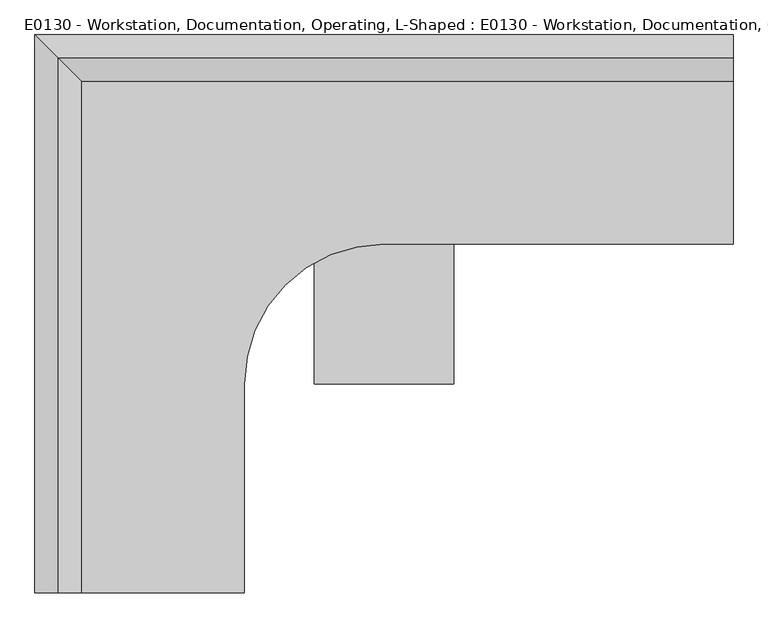
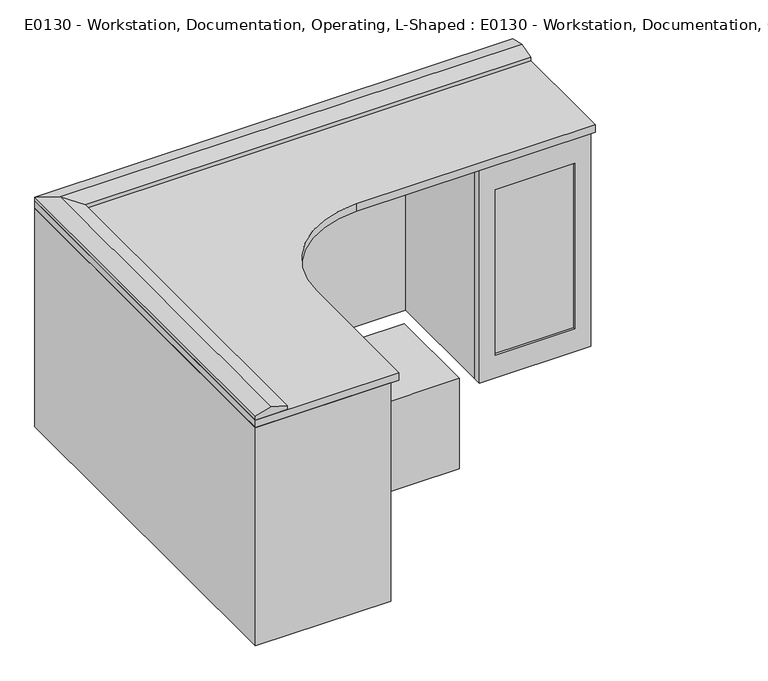
"""IFC4 building model written with IfcOpenShell, lengths in millimetres: proxy geometry, E0130 - Workstation, Documentation, Operating, L-Shaped : E0130 - Workstation, Documentation, Operating, L-Shaped."""

import ifcopenshell
import ifcopenshell.guid

model = None  # the IFC model being written
_history = None  # IfcOwnerHistory: only IFC2X3 demands one
_inside = {}  # id of a spatial element -> (the spatial element, [elements in it])
_under = {}  # id of a project, library or spatial element -> (it, [spatial elements below it])
_declared = {}  # id of a project -> (the project, [libraries it declares])
_typed = {}  # id of a type object -> (the type object, [elements of that type])
_made_of = {}  # id of a material, layer set ... -> (it, [elements and type objects made of it])


def new_model(schema):
    """Start an empty IFC model of exactly this schema.

    Asked for "IFC4X3", IfcOpenShell would pick the latest addendum, in which some entities
    have other attributes; the version numbers below select the first issue.
    IFC2X3 requires an IfcOwnerHistory on every rooted entity: one is made here for all.
    """
    global model, _history
    if schema == "IFC4X3":
        model = ifcopenshell.file(schema_version=(4, 3, 0, 0))
    else:
        model = ifcopenshell.file(schema=schema)
    _inside.clear()
    _under.clear()
    _declared.clear()
    _typed.clear()
    _made_of.clear()
    _history = None
    if model.schema == "IFC2X3":
        org = make("IfcOrganization", Name="unknown")
        user = make(
            "IfcPersonAndOrganization",
            ThePerson=make("IfcPerson", FamilyName="unknown"),
            TheOrganization=org,
        )
        app = make(
            "IfcApplication",
            ApplicationDeveloper=org,
            Version="unknown",
            ApplicationFullName="unknown",
            ApplicationIdentifier="unknown",
        )
        _history = make(
            "IfcOwnerHistory",
            OwningUser=user,
            OwningApplication=app,
            ChangeAction="ADDED",
            CreationDate=0,
        )
    return model


def make(cls, **values):
    """One entity of the class cls with the attributes given. An attribute that is None is left unset."""
    return model.create_entity(
        cls, **{name: value for name, value in values.items() if value is not None}
    )


def rooted(cls, **values):
    """An entity with a GlobalId (a new one), such as an element, a storey or a relation."""
    return make(cls, GlobalId=ifcopenshell.guid.new(), OwnerHistory=_history, **values)


def si_unit(unit_type, name, prefix=None):
    """IfcSIUnit, for example si_unit("LENGTHUNIT", "METRE", prefix="MILLI")."""
    return make("IfcSIUnit", UnitType=unit_type, Prefix=prefix, Name=name)


def assignment(units):
    """IfcUnitAssignment: the units of a project."""
    return None if units is None else make("IfcUnitAssignment", Units=units)


def point(xyz):
    """IfcCartesianPoint."""
    return None if xyz is None else make("IfcCartesianPoint", Coordinates=xyz)


def direction(xyz):
    """IfcDirection."""
    return None if xyz is None else make("IfcDirection", DirectionRatios=xyz)


def frame(location, z_axis=None, x_axis=None):
    """IfcAxis2Placement3D, a coordinate frame: its origin and axes. An axis left out is left unset."""
    return make(
        "IfcAxis2Placement3D",
        Location=point(location),
        Axis=direction(z_axis),
        RefDirection=direction(x_axis),
    )


def frame_2d(location, x_axis=None):
    """IfcAxis2Placement2D, a coordinate frame in the plane: its origin and x axis."""
    return make(
        "IfcAxis2Placement2D", Location=point(location), RefDirection=direction(x_axis)
    )


def origin():
    """The frame at (0, 0, 0) with its axes left unset."""
    return frame((0.0, 0.0, 0.0))


def origin_with_axes():
    """The frame at (0, 0, 0) with the z axis (0, 0, 1) and the x axis (1, 0, 0) written out."""
    return frame((0.0, 0.0, 0.0), z_axis=(0.0, 0.0, 1.0), x_axis=(1.0, 0.0, 0.0))


def place(relative_to, where):
    """IfcLocalPlacement: puts the frame where relative to a parent placement (None: the world)."""
    return make(
        "IfcLocalPlacement", PlacementRelTo=relative_to, RelativePlacement=where
    )


def context(
    kind, dimensions, precision=None, world=None, true_north=None, identifier=None
):
    """IfcGeometricRepresentationContext, for example the 3D "Model" context."""
    return make(
        "IfcGeometricRepresentationContext",
        ContextIdentifier=identifier,
        ContextType=kind,
        CoordinateSpaceDimension=dimensions,
        Precision=precision,
        WorldCoordinateSystem=world,
        TrueNorth=true_north,
    )


def project(units=None, contexts=None):
    """IfcProject with its units and contexts."""
    return rooted(
        "IfcProject",
        Name="project",
        RepresentationContexts=contexts,
        UnitsInContext=assignment(units),
    )


def spatial(cls, under=None, at=None, **own):
    """A site, building, storey or space (cls), placed at a placement, below another one or the project."""
    s = rooted(cls, ObjectPlacement=at, **own)
    if under is not None:
        _under.setdefault(under.id(), (under, []))[1].append(s)
    return s


def polyline(points):
    """IfcPolyline through the points."""
    return make("IfcPolyline", Points=[point(p) for p in points])


def circle_curve(where, radius):
    """IfcCircle in the frame where."""
    return make("IfcCircle", Position=where, Radius=radius)


def trimmed(basis, trim1, trim2, sense, master):
    """IfcTrimmedCurve: the piece of a basis curve between two trims."""
    return make(
        "IfcTrimmedCurve",
        BasisCurve=basis,
        Trim1=trim1,
        Trim2=trim2,
        SenseAgreement=sense,
        MasterRepresentation=master,
    )


def segment(curve, same_sense, transition):
    """IfcCompositeCurveSegment."""
    return make(
        "IfcCompositeCurveSegment",
        Transition=transition,
        SameSense=same_sense,
        ParentCurve=curve,
    )


def composite_curve(segments, self_intersect=None):
    """IfcCompositeCurve: segments joined end to end."""
    return make("IfcCompositeCurve", Segments=segments, SelfIntersect=self_intersect)


def outline(outer, holes=None, kind="AREA"):
    """IfcArbitraryClosedProfileDef: a profile drawn as a closed curve; with holes, ...WithVoids."""
    if holes is None:
        return make("IfcArbitraryClosedProfileDef", ProfileType=kind, OuterCurve=outer)
    return make(
        "IfcArbitraryProfileDefWithVoids",
        ProfileType=kind,
        OuterCurve=outer,
        InnerCurves=holes,
    )


def extrude(swept, where, along, depth):
    """IfcExtrudedAreaSolid: the profile swept, set in the frame where, extruded along a direction by depth."""
    return make(
        "IfcExtrudedAreaSolid",
        SweptArea=swept,
        Position=where,
        ExtrudedDirection=direction(along),
        Depth=depth,
    )


def faces_of(points, faces, orient=None, outer=None):
    """IfcFace entities. A face is a list of loops; a loop is a list of indices into points, from 0.

    orient and outer hold one flag for each loop. By default every Orientation is true, the
    first loop of a face is its IfcFaceOuterBound and the others are IfcFaceBound.
    """
    made = []
    for i, loops in enumerate(faces):
        bounds = []
        for j, loop in enumerate(loops):
            is_outer = j == 0 if outer is None else outer[i][j]
            bounds.append(
                make(
                    "IfcFaceOuterBound" if is_outer else "IfcFaceBound",
                    Bound=make("IfcPolyLoop", Polygon=[points[k] for k in loop]),
                    Orientation=True if orient is None else orient[i][j],
                )
            )
        made.append(make("IfcFace", Bounds=bounds))
    return made


def faceted_brep(points, faces, orient=None, outer=None, voids=None):
    """IfcFacetedBrep: a solid bounded by flat faces; with voids (closed shells), ...WithVoids."""
    shared = [point(p) for p in points]
    hull = make("IfcClosedShell", CfsFaces=faces_of(shared, faces, orient, outer))
    if voids is None:
        return make("IfcFacetedBrep", Outer=hull)
    return make(
        "IfcFacetedBrepWithVoids",
        Outer=hull,
        Voids=[
            make(cls, CfsFaces=faces_of(shared, fs, o, b)) for cls, fs, o, b in voids
        ],
    )


def shape(context_of_items, identifier, shape_type, items):
    """IfcShapeRepresentation: the items that make up one representation, for example the "Body"."""
    return make(
        "IfcShapeRepresentation",
        ContextOfItems=context_of_items,
        RepresentationIdentifier=identifier,
        RepresentationType=shape_type,
        Items=items,
    )


def source(mapping_origin, context_of_items, identifier, shape_type, items):
    """IfcRepresentationMap: a shape defined once, which mapped items show again and again."""
    return make(
        "IfcRepresentationMap",
        MappingOrigin=mapping_origin,
        MappedRepresentation=shape(context_of_items, identifier, shape_type, items),
    )


def transform(
    local_origin,
    x_axis=None,
    y_axis=None,
    z_axis=None,
    scale=None,
    scale2=None,
    scale3=None,
    uniform=True,
):
    """IfcCartesianTransformationOperator3D, or its non-uniform kind. x_axis, y_axis, z_axis: its Axis1, 2, 3."""
    if uniform:
        return make(
            "IfcCartesianTransformationOperator3D",
            Axis1=direction(x_axis),
            Axis2=direction(y_axis),
            LocalOrigin=point(local_origin),
            Scale=scale,
            Axis3=direction(z_axis),
        )
    return make(
        "IfcCartesianTransformationOperator3DnonUniform",
        Axis1=direction(x_axis),
        Axis2=direction(y_axis),
        LocalOrigin=point(local_origin),
        Scale=scale,
        Axis3=direction(z_axis),
        Scale2=scale2,
        Scale3=scale3,
    )


def mapped(mapping_source, mapping_target):
    """IfcMappedItem: shows the shape of a source again, moved by a transform."""
    return make(
        "IfcMappedItem", MappingSource=mapping_source, MappingTarget=mapping_target
    )


def made_of(thing, what):
    """Note that an element or type object is made of a material, layer set ...; save() writes the relation."""
    if what is not None:
        _made_of.setdefault(what.id(), (what, []))[1].append(thing)
    return thing


def element(
    cls,
    number,
    at=None,
    inside=None,
    cuts=None,
    type_object=None,
    material=None,
    context=None,
    identifier="Body",
    shape_type=None,
    held_by="IfcProductDefinitionShape",
    body=None,
    shapes=None,
    **own,
):
    """One element of the class cls, such as IfcWall. Its Tag is "e" and its number.

    at: its placement. inside: the storey or other place that contains it. cuts: it is an
    opening in that element (IfcRelVoidsElement). A single representation is given by context,
    identifier, shape_type and body (its items); several are given by shapes. held_by: the class
    of the entity that holds the representations. save() writes the other relations.
    """
    e = rooted(cls, Tag="e%d" % number, ObjectPlacement=at, **own)
    if body is not None:
        shapes = [shape(context, identifier, shape_type, body)]
    if shapes is not None:
        e.Representation = make(held_by, Representations=shapes)
    if inside is not None:
        _inside.setdefault(inside.id(), (inside, []))[1].append(e)
    if cuts is not None:
        rooted(
            "IfcRelVoidsElement", RelatingBuildingElement=cuts, RelatedOpeningElement=e
        )
    if type_object is not None:
        _typed.setdefault(type_object.id(), (type_object, []))[1].append(e)
    return made_of(e, material)


def aggregate(whole, parts):
    """IfcRelAggregates: a whole, such as a stair, and the parts it consists of."""
    return rooted("IfcRelAggregates", RelatingObject=whole, RelatedObjects=parts)


def save(model, path):
    """Write the relations noted so far, then the file.

    IfcRelAggregates (storeys below a building ...), IfcRelContainedInSpatialStructure (elements
    in a storey), IfcRelDefinesByType, IfcRelAssociatesMaterial and IfcRelDeclares: one each for
    every whole, place, type object, material and project.
    """
    for whole, parts in _under.values():
        aggregate(whole, parts)
    for where, things in _inside.values():
        rooted(
            "IfcRelContainedInSpatialStructure",
            RelatedElements=things,
            RelatingStructure=where,
        )
    for kind, things in _typed.values():
        rooted("IfcRelDefinesByType", RelatedObjects=things, RelatingType=kind)
    for what, things in _made_of.values():
        rooted("IfcRelAssociatesMaterial", RelatedObjects=things, RelatingMaterial=what)
    for by, libraries in _declared.values():
        rooted("IfcRelDeclares", RelatingContext=by, RelatedDefinitions=libraries)
    model.write(path)


def e0130_workstation_documentation_operating_l_shaped_e0130_dad7d897(model_context):
    return source(origin(), model_context, "Body", "SolidModel", [
        extrude(outline(polyline([(711.2, 184.9965826), (457.2, 184.9965826), (457.2, 193.8982967), (711.2, 193.8982967), (711.2, 184.9965826)])), frame((0.0, 0.0, 76.2), z_axis=(0.0, 0.0, 1.0), x_axis=(1.0, 0.0, 0.0)), (0.0, 0.0, 1.0), 558.8),
        extrude(outline(polyline([(736.6, 762.0), (736.6, 406.4), (0.0, 406.4), (0.0, 762.0), (736.6, 762.0)]), holes=[polyline([(635.0, 711.2), (76.2, 711.2), (76.2, 457.2), (635.0, 457.2), (635.0, 711.2)])]), frame((0.0, 177.8, 0.0), z_axis=(0.0, 1.0, 0.0), x_axis=(0.0, 0.0, 1.0)), (0.0, 0.0, 1.0), 25.4),
        faceted_brep([(-660.4, -609.6, 762.0), (-660.4, -609.6, 774.7), (-711.2, -609.6, 788.311819), (-762.0, -609.6, 774.7), (-762.0, -609.6, 762.0), (-762.0, 609.6, 762.0), (762.0, 609.6, 762.0), (762.0, 508.0, 762.0), (-660.4, 508.0, 762.0), (762.0, 609.6, 774.7), (762.0, 558.8, 788.311819), (762.0, 508.0, 774.7), (-660.4, 508.0, 774.7), (-711.2, 558.8, 788.311819), (-762.0, 609.6, 774.7)], [[[0, 1, 2, 3, 4]], [[0, 4, 5, 6, 7, 8]], [[7, 6, 9, 10, 11]], [[1, 0, 8, 12]], [[2, 1, 12, 13]], [[3, 2, 13, 14]], [[4, 3, 14, 5]], [[12, 8, 7, 11]], [[13, 12, 11, 10]], [[14, 13, 10, 9]], [[5, 14, 9, 6]]]),
        extrude(outline(polyline([(431.8, 558.8), (431.8, 203.2), (406.4, 203.2), (406.4, 584.2), (736.6, 584.2), (736.6, 558.8), (431.8, 558.8)])), origin_with_axes(), (0.0, 0.0, 1.0), 736.6),
        extrude(outline(polyline([(-762.0, 609.6), (762.0, 609.6), (762.0, 203.2), (736.6, 203.2), (736.6, 584.2), (-736.6, 584.2), (-736.6, -584.2), (-330.2, -584.2), (-330.2, -609.6), (-762.0, -609.6), (-762.0, 609.6)])), origin_with_axes(), (0.0, 0.0, 1.0), 736.6),
        extrude(outline(composite_curve([segment(polyline([(762.0, 609.6), (762.0, 152.4), (0.0, 152.4)]), True, "CONTINUOUS"), segment(trimmed(circle_curve(frame_2d((0.0, -152.4)), 304.8), [point((0.0, 152.4))], [point((-304.8, -152.4))], True, "CARTESIAN"), True, "CONTINUOUS"), segment(polyline([(-304.8, -152.4), (-304.8, -609.6), (-762.0, -609.6), (-762.0, 609.6), (762.0, 609.6)]), True, "CONTINUOUS")], self_intersect=False)), frame((0.0, 0.0, 736.6), z_axis=(0.0, 0.0, 1.0), x_axis=(1.0, 0.0, 0.0)), (0.0, 0.0, 1.0), 25.4),
        extrude(outline(polyline([(-152.4, 152.4), (152.4, 152.4), (152.4, -152.4), (-152.4, -152.4), (-152.4, 0.0), (-152.4, 152.4)])), origin_with_axes(), (0.0, 0.0, 1.0), 304.8),
    ])


if __name__ == "__main__":
    model = new_model("IFC4")
    model_context = context("Model", 3, world=origin())
    ifc_project = project(units=[si_unit("LENGTHUNIT", "METRE", prefix="MILLI")], contexts=[model_context])
    site = spatial("IfcSite", under=ifc_project)
    building = spatial("IfcBuilding", under=site)
    placement = place(None, origin())
    e0130_workstation_documentation_operating_l_shaped_e0130_shape = e0130_workstation_documentation_operating_l_shaped_e0130_dad7d897(model_context)
    element("IfcBuildingElementProxy", 1, Name="E0130 - Workstation, Documentation, Operating, L-Shaped : E0130 - Workstation, Documentation, Operating, L-Shaped", ObjectType="E0130 - Workstation, Documentation, Operating, L-Shaped : E0130 - Workstation, Documentation, Operating, L-Shaped", at=placement, inside=building, context=model_context, shape_type="MappedRepresentation", body=[
        mapped(e0130_workstation_documentation_operating_l_shaped_e0130_shape, transform((0.0, 0.0, 0.0), x_axis=(1.0, 0.0, 0.0), y_axis=(0.0, 1.0, 0.0), z_axis=(0.0, 0.0, 1.0))),
    ])
    save(model, "model.ifc")

# Revit data of these elements
# Type "E0130 - Workstation, Documentation, Operating, L-Shaped : E0130 - Workstation, Documentation, Operating, L-Shaped"
#   JSN = "E0130"
#   Nomenclature = "Workstation, Documentation, OR, L-Shaped"
#   UTIL_1_WaterDrain = "-"
#   UTIL_2_Elec = "A"
#   UTIL_3_MedGas = "-"
#   UTIL_4_MiscGas = "-"
#   UTIL_5_NonMedGas = "-"
#   UTIL_6_Misc = "-"
#   Utility_6 = "-"
#   Utility_5 = "-"
#   Utility_4 = "-"
#   Utility_3 = "-"
#   Utility_2 = "A"
#   Utility_1 = "-"
#   Unit_Issue = "EA"
#   Price_Date = "07/08/2013"
#   Nomenclature = "Workstation, Documentation, OR, L-Shaped"
#   NSN = "6515"
#   Location [instance default] = ""
#   JSN_Name = "E0130"
#   Hertz_swit = "0"
#   Hertz_dep = "1"
#   Hertz = "60"
#   Desc = "A 60\" L-shaped documentation workstation for use in the OR. The workstation may be either a right or left hand configuration. It will consist of a back panel with dry-erase whiteboard, marker storage tray, optional mounting for monitors, an articulating task light and a keyboard tray. The workstation will also include electrical, data, telecommunication and video cable channels and wire ways to support various applications. An integrated power source will be desk-top mounted and provide two electrical outlets, a telephone jack and a computer network jack."
#   CAT_VA = "-"
#   CAT_Navy = "C"
#   CAT_IHS = "C"
#   CAT_Army = "C"
#   CAT_AF = "-"
#   BTUPerHour = "0"
#   Width_IN = 66
#   Weight_AV = 0
#   Watts2 = 0
#   Watts1 = 240
#   Volts2 = 0
#   Volts1 = 120
#   Phase2 = 0
#   Phase1 = 1
#   Height_IN = 55
#   Depth_IN = 54
#   Amps2 = 0
#   Amps1 = 2
# Element 1 (IfcBuildingElementProxy, "E0130 - Workstation, Documentation, Operating, L-Shaped : E0130 - Workstation, Documentation, Operating, L-Shaped")
#   Materials on its faces: "EquipSpace", "Glass"
# Materials
#   "EquipSpace": class "Unassigned", colour RGB 221 217 195, transparency 0.5
#   "Glass": class "Glass", colour RGB 0 128 192, transparency 0.75
